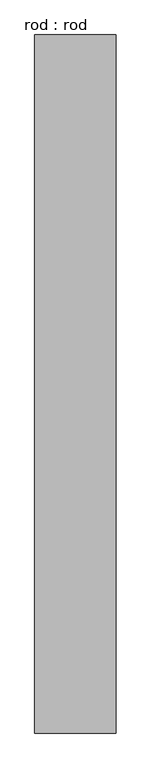
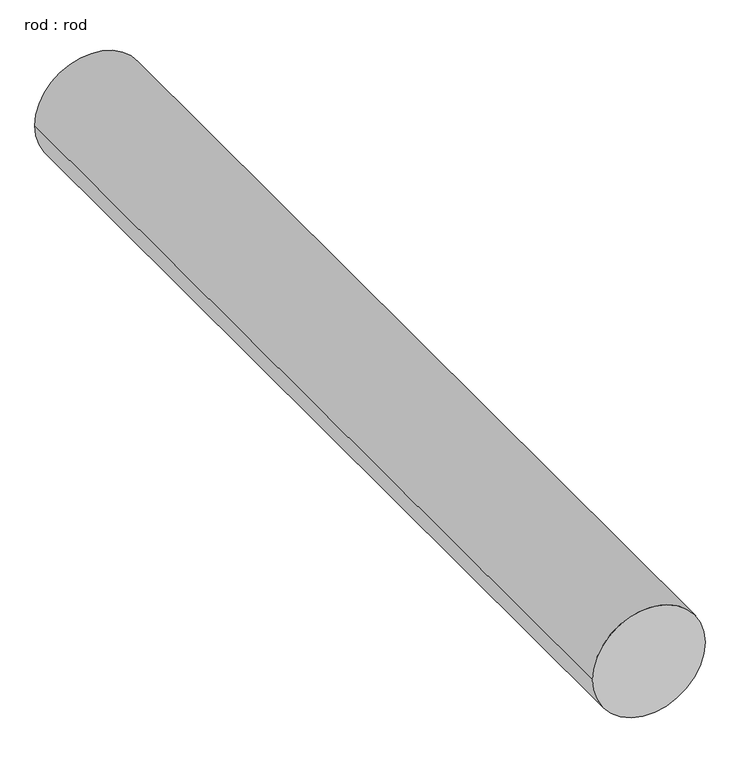
"""IFC4 building model written with IfcOpenShell, lengths in millimetres: proxy geometry, rod : rod."""

import ifcopenshell
import ifcopenshell.guid

model = None  # the IFC model being written
_history = None  # IfcOwnerHistory: only IFC2X3 demands one
_inside = {}  # id of a spatial element -> (the spatial element, [elements in it])
_under = {}  # id of a project, library or spatial element -> (it, [spatial elements below it])
_declared = {}  # id of a project -> (the project, [libraries it declares])
_typed = {}  # id of a type object -> (the type object, [elements of that type])
_made_of = {}  # id of a material, layer set ... -> (it, [elements and type objects made of it])


def new_model(schema):
    """Start an empty IFC model of exactly this schema.

    Asked for "IFC4X3", IfcOpenShell would pick the latest addendum, in which some entities
    have other attributes; the version numbers below select the first issue.
    IFC2X3 requires an IfcOwnerHistory on every rooted entity: one is made here for all.
    """
    global model, _history
    if schema == "IFC4X3":
        model = ifcopenshell.file(schema_version=(4, 3, 0, 0))
    else:
        model = ifcopenshell.file(schema=schema)
    _inside.clear()
    _under.clear()
    _declared.clear()
    _typed.clear()
    _made_of.clear()
    _history = None
    if model.schema == "IFC2X3":
        org = make("IfcOrganization", Name="unknown")
        user = make(
            "IfcPersonAndOrganization",
            ThePerson=make("IfcPerson", FamilyName="unknown"),
            TheOrganization=org,
        )
        app = make(
            "IfcApplication",
            ApplicationDeveloper=org,
            Version="unknown",
            ApplicationFullName="unknown",
            ApplicationIdentifier="unknown",
        )
        _history = make(
            "IfcOwnerHistory",
            OwningUser=user,
            OwningApplication=app,
            ChangeAction="ADDED",
            CreationDate=0,
        )
    return model


def make(cls, **values):
    """One entity of the class cls with the attributes given. An attribute that is None is left unset."""
    return model.create_entity(
        cls, **{name: value for name, value in values.items() if value is not None}
    )


def rooted(cls, **values):
    """An entity with a GlobalId (a new one), such as an element, a storey or a relation."""
    return make(cls, GlobalId=ifcopenshell.guid.new(), OwnerHistory=_history, **values)


def si_unit(unit_type, name, prefix=None):
    """IfcSIUnit, for example si_unit("LENGTHUNIT", "METRE", prefix="MILLI")."""
    return make("IfcSIUnit", UnitType=unit_type, Prefix=prefix, Name=name)


def assignment(units):
    """IfcUnitAssignment: the units of a project."""
    return None if units is None else make("IfcUnitAssignment", Units=units)


def point(xyz):
    """IfcCartesianPoint."""
    return None if xyz is None else make("IfcCartesianPoint", Coordinates=xyz)


def direction(xyz):
    """IfcDirection."""
    return None if xyz is None else make("IfcDirection", DirectionRatios=xyz)


def frame(location, z_axis=None, x_axis=None):
    """IfcAxis2Placement3D, a coordinate frame: its origin and axes. An axis left out is left unset."""
    return make(
        "IfcAxis2Placement3D",
        Location=point(location),
        Axis=direction(z_axis),
        RefDirection=direction(x_axis),
    )


def frame_2d(location, x_axis=None):
    """IfcAxis2Placement2D, a coordinate frame in the plane: its origin and x axis."""
    return make(
        "IfcAxis2Placement2D", Location=point(location), RefDirection=direction(x_axis)
    )


def origin():
    """The frame at (0, 0, 0) with its axes left unset."""
    return frame((0.0, 0.0, 0.0))


def place(relative_to, where):
    """IfcLocalPlacement: puts the frame where relative to a parent placement (None: the world)."""
    return make(
        "IfcLocalPlacement", PlacementRelTo=relative_to, RelativePlacement=where
    )


def context(
    kind, dimensions, precision=None, world=None, true_north=None, identifier=None
):
    """IfcGeometricRepresentationContext, for example the 3D "Model" context."""
    return make(
        "IfcGeometricRepresentationContext",
        ContextIdentifier=identifier,
        ContextType=kind,
        CoordinateSpaceDimension=dimensions,
        Precision=precision,
        WorldCoordinateSystem=world,
        TrueNorth=true_north,
    )


def project(units=None, contexts=None):
    """IfcProject with its units and contexts."""
    return rooted(
        "IfcProject",
        Name="project",
        RepresentationContexts=contexts,
        UnitsInContext=assignment(units),
    )


def spatial(cls, under=None, at=None, **own):
    """A site, building, storey or space (cls), placed at a placement, below another one or the project."""
    s = rooted(cls, ObjectPlacement=at, **own)
    if under is not None:
        _under.setdefault(under.id(), (under, []))[1].append(s)
    return s


def circle_curve(where, radius):
    """IfcCircle in the frame where."""
    return make("IfcCircle", Position=where, Radius=radius)


def trimmed(basis, trim1, trim2, sense, master):
    """IfcTrimmedCurve: the piece of a basis curve between two trims."""
    return make(
        "IfcTrimmedCurve",
        BasisCurve=basis,
        Trim1=trim1,
        Trim2=trim2,
        SenseAgreement=sense,
        MasterRepresentation=master,
    )


def segment(curve, same_sense, transition):
    """IfcCompositeCurveSegment."""
    return make(
        "IfcCompositeCurveSegment",
        Transition=transition,
        SameSense=same_sense,
        ParentCurve=curve,
    )


def composite_curve(segments, self_intersect=None):
    """IfcCompositeCurve: segments joined end to end."""
    return make("IfcCompositeCurve", Segments=segments, SelfIntersect=self_intersect)


def outline(outer, holes=None, kind="AREA"):
    """IfcArbitraryClosedProfileDef: a profile drawn as a closed curve; with holes, ...WithVoids."""
    if holes is None:
        return make("IfcArbitraryClosedProfileDef", ProfileType=kind, OuterCurve=outer)
    return make(
        "IfcArbitraryProfileDefWithVoids",
        ProfileType=kind,
        OuterCurve=outer,
        InnerCurves=holes,
    )


def extrude(swept, where, along, depth):
    """IfcExtrudedAreaSolid: the profile swept, set in the frame where, extruded along a direction by depth."""
    return make(
        "IfcExtrudedAreaSolid",
        SweptArea=swept,
        Position=where,
        ExtrudedDirection=direction(along),
        Depth=depth,
    )


def shape(context_of_items, identifier, shape_type, items):
    """IfcShapeRepresentation: the items that make up one representation, for example the "Body"."""
    return make(
        "IfcShapeRepresentation",
        ContextOfItems=context_of_items,
        RepresentationIdentifier=identifier,
        RepresentationType=shape_type,
        Items=items,
    )


def source(mapping_origin, context_of_items, identifier, shape_type, items):
    """IfcRepresentationMap: a shape defined once, which mapped items show again and again."""
    return make(
        "IfcRepresentationMap",
        MappingOrigin=mapping_origin,
        MappedRepresentation=shape(context_of_items, identifier, shape_type, items),
    )


def transform(
    local_origin,
    x_axis=None,
    y_axis=None,
    z_axis=None,
    scale=None,
    scale2=None,
    scale3=None,
    uniform=True,
):
    """IfcCartesianTransformationOperator3D, or its non-uniform kind. x_axis, y_axis, z_axis: its Axis1, 2, 3."""
    if uniform:
        return make(
            "IfcCartesianTransformationOperator3D",
            Axis1=direction(x_axis),
            Axis2=direction(y_axis),
            LocalOrigin=point(local_origin),
            Scale=scale,
            Axis3=direction(z_axis),
        )
    return make(
        "IfcCartesianTransformationOperator3DnonUniform",
        Axis1=direction(x_axis),
        Axis2=direction(y_axis),
        LocalOrigin=point(local_origin),
        Scale=scale,
        Axis3=direction(z_axis),
        Scale2=scale2,
        Scale3=scale3,
    )


def mapped(mapping_source, mapping_target):
    """IfcMappedItem: shows the shape of a source again, moved by a transform."""
    return make(
        "IfcMappedItem", MappingSource=mapping_source, MappingTarget=mapping_target
    )


def made_of(thing, what):
    """Note that an element or type object is made of a material, layer set ...; save() writes the relation."""
    if what is not None:
        _made_of.setdefault(what.id(), (what, []))[1].append(thing)
    return thing


def element(
    cls,
    number,
    at=None,
    inside=None,
    cuts=None,
    type_object=None,
    material=None,
    context=None,
    identifier="Body",
    shape_type=None,
    held_by="IfcProductDefinitionShape",
    body=None,
    shapes=None,
    **own,
):
    """One element of the class cls, such as IfcWall. Its Tag is "e" and its number.

    at: its placement. inside: the storey or other place that contains it. cuts: it is an
    opening in that element (IfcRelVoidsElement). A single representation is given by context,
    identifier, shape_type and body (its items); several are given by shapes. held_by: the class
    of the entity that holds the representations. save() writes the other relations.
    """
    e = rooted(cls, Tag="e%d" % number, ObjectPlacement=at, **own)
    if body is not None:
        shapes = [shape(context, identifier, shape_type, body)]
    if shapes is not None:
        e.Representation = make(held_by, Representations=shapes)
    if inside is not None:
        _inside.setdefault(inside.id(), (inside, []))[1].append(e)
    if cuts is not None:
        rooted(
            "IfcRelVoidsElement", RelatingBuildingElement=cuts, RelatedOpeningElement=e
        )
    if type_object is not None:
        _typed.setdefault(type_object.id(), (type_object, []))[1].append(e)
    return made_of(e, material)


def aggregate(whole, parts):
    """IfcRelAggregates: a whole, such as a stair, and the parts it consists of."""
    return rooted("IfcRelAggregates", RelatingObject=whole, RelatedObjects=parts)


def save(model, path):
    """Write the relations noted so far, then the file.

    IfcRelAggregates (storeys below a building ...), IfcRelContainedInSpatialStructure (elements
    in a storey), IfcRelDefinesByType, IfcRelAssociatesMaterial and IfcRelDeclares: one each for
    every whole, place, type object, material and project.
    """
    for whole, parts in _under.values():
        aggregate(whole, parts)
    for where, things in _inside.values():
        rooted(
            "IfcRelContainedInSpatialStructure",
            RelatedElements=things,
            RelatingStructure=where,
        )
    for kind, things in _typed.values():
        rooted("IfcRelDefinesByType", RelatedObjects=things, RelatingType=kind)
    for what, things in _made_of.values():
        rooted("IfcRelAssociatesMaterial", RelatedObjects=things, RelatingMaterial=what)
    for by, libraries in _declared.values():
        rooted("IfcRelDeclares", RelatingContext=by, RelatedDefinitions=libraries)
    model.write(path)


def rod_rod_c2f5ad5a(model_context):
    return source(origin(), model_context, "Body", "SweptSolid", [
        extrude(outline(composite_curve([segment(trimmed(circle_curve(frame_2d((0.0108462, 0.0)), 200.0), [point((0.0108462, 200.0))], [point((0.0108462, -200.0))], False, "CARTESIAN"), True, "CONTINUOUS"), segment(trimmed(circle_curve(frame_2d((0.0108462, 0.0)), 200.0), [point((0.0108462, -200.0))], [point((0.0108462, 200.0))], False, "CARTESIAN"), True, "CONTINUOUS")], self_intersect=False)), frame((0.0, 2378.4429011, 0.0), z_axis=(0.0, 1.0, 0.0), x_axis=(0.0, 0.0, 1.0)), (0.0, 0.0, 1.0), 3428.5714286),
    ])


if __name__ == "__main__":
    model = new_model("IFC4")
    model_context = context("Model", 3, world=origin())
    ifc_project = project(units=[si_unit("LENGTHUNIT", "METRE", prefix="MILLI")], contexts=[model_context])
    site = spatial("IfcSite", under=ifc_project)
    building = spatial("IfcBuilding", under=site)
    placement = place(None, origin())
    rod_rod_shape = rod_rod_c2f5ad5a(model_context)
    element("IfcBuildingElementProxy", 1, Name="rod : rod", ObjectType="rod : rod", at=placement, inside=building, context=model_context, shape_type="MappedRepresentation", body=[
        mapped(rod_rod_shape, transform((0.0, 0.0, 0.0), x_axis=(1.0, 0.0, 0.0), y_axis=(0.0, 1.0, 0.0), z_axis=(0.0, 0.0, 1.0))),
    ])
    save(model, "model.ifc")

# Revit data of these elements
# Type "rod : rod"
#   Default Elevation = 0
